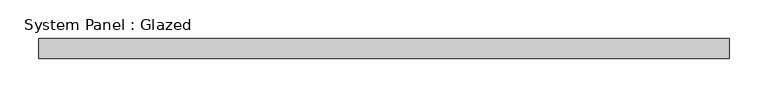
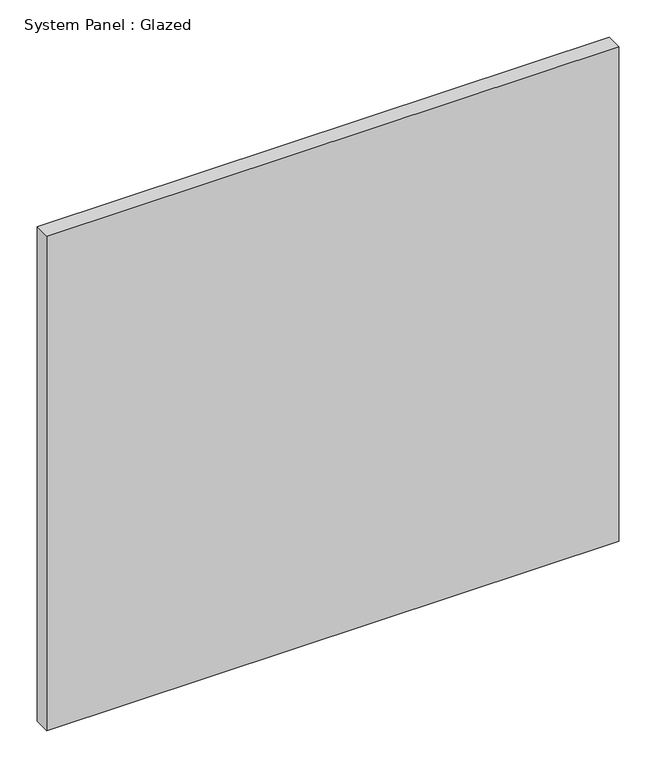
"""IFC4 building model written with IfcOpenShell, lengths in millimetres: plate geometry, System Panel : Glazed."""

import ifcopenshell
import ifcopenshell.guid

model = None  # the IFC model being written
_history = None  # IfcOwnerHistory: only IFC2X3 demands one
_inside = {}  # id of a spatial element -> (the spatial element, [elements in it])
_under = {}  # id of a project, library or spatial element -> (it, [spatial elements below it])
_declared = {}  # id of a project -> (the project, [libraries it declares])
_typed = {}  # id of a type object -> (the type object, [elements of that type])
_made_of = {}  # id of a material, layer set ... -> (it, [elements and type objects made of it])


def new_model(schema):
    """Start an empty IFC model of exactly this schema.

    Asked for "IFC4X3", IfcOpenShell would pick the latest addendum, in which some entities
    have other attributes; the version numbers below select the first issue.
    IFC2X3 requires an IfcOwnerHistory on every rooted entity: one is made here for all.
    """
    global model, _history
    if schema == "IFC4X3":
        model = ifcopenshell.file(schema_version=(4, 3, 0, 0))
    else:
        model = ifcopenshell.file(schema=schema)
    _inside.clear()
    _under.clear()
    _declared.clear()
    _typed.clear()
    _made_of.clear()
    _history = None
    if model.schema == "IFC2X3":
        org = make("IfcOrganization", Name="unknown")
        user = make(
            "IfcPersonAndOrganization",
            ThePerson=make("IfcPerson", FamilyName="unknown"),
            TheOrganization=org,
        )
        app = make(
            "IfcApplication",
            ApplicationDeveloper=org,
            Version="unknown",
            ApplicationFullName="unknown",
            ApplicationIdentifier="unknown",
        )
        _history = make(
            "IfcOwnerHistory",
            OwningUser=user,
            OwningApplication=app,
            ChangeAction="ADDED",
            CreationDate=0,
        )
    return model


def make(cls, **values):
    """One entity of the class cls with the attributes given. An attribute that is None is left unset."""
    return model.create_entity(
        cls, **{name: value for name, value in values.items() if value is not None}
    )


def rooted(cls, **values):
    """An entity with a GlobalId (a new one), such as an element, a storey or a relation."""
    return make(cls, GlobalId=ifcopenshell.guid.new(), OwnerHistory=_history, **values)


def si_unit(unit_type, name, prefix=None):
    """IfcSIUnit, for example si_unit("LENGTHUNIT", "METRE", prefix="MILLI")."""
    return make("IfcSIUnit", UnitType=unit_type, Prefix=prefix, Name=name)


def assignment(units):
    """IfcUnitAssignment: the units of a project."""
    return None if units is None else make("IfcUnitAssignment", Units=units)


def point(xyz):
    """IfcCartesianPoint."""
    return None if xyz is None else make("IfcCartesianPoint", Coordinates=xyz)


def direction(xyz):
    """IfcDirection."""
    return None if xyz is None else make("IfcDirection", DirectionRatios=xyz)


def frame(location, z_axis=None, x_axis=None):
    """IfcAxis2Placement3D, a coordinate frame: its origin and axes. An axis left out is left unset."""
    return make(
        "IfcAxis2Placement3D",
        Location=point(location),
        Axis=direction(z_axis),
        RefDirection=direction(x_axis),
    )


def origin():
    """The frame at (0, 0, 0) with its axes left unset."""
    return frame((0.0, 0.0, 0.0))


def origin_with_axes():
    """The frame at (0, 0, 0) with the z axis (0, 0, 1) and the x axis (1, 0, 0) written out."""
    return frame((0.0, 0.0, 0.0), z_axis=(0.0, 0.0, 1.0), x_axis=(1.0, 0.0, 0.0))


def place(relative_to, where):
    """IfcLocalPlacement: puts the frame where relative to a parent placement (None: the world)."""
    return make(
        "IfcLocalPlacement", PlacementRelTo=relative_to, RelativePlacement=where
    )


def context(
    kind, dimensions, precision=None, world=None, true_north=None, identifier=None
):
    """IfcGeometricRepresentationContext, for example the 3D "Model" context."""
    return make(
        "IfcGeometricRepresentationContext",
        ContextIdentifier=identifier,
        ContextType=kind,
        CoordinateSpaceDimension=dimensions,
        Precision=precision,
        WorldCoordinateSystem=world,
        TrueNorth=true_north,
    )


def project(units=None, contexts=None):
    """IfcProject with its units and contexts."""
    return rooted(
        "IfcProject",
        Name="project",
        RepresentationContexts=contexts,
        UnitsInContext=assignment(units),
    )


def spatial(cls, under=None, at=None, **own):
    """A site, building, storey or space (cls), placed at a placement, below another one or the project."""
    s = rooted(cls, ObjectPlacement=at, **own)
    if under is not None:
        _under.setdefault(under.id(), (under, []))[1].append(s)
    return s


def polyline(points):
    """IfcPolyline through the points."""
    return make("IfcPolyline", Points=[point(p) for p in points])


def outline(outer, holes=None, kind="AREA"):
    """IfcArbitraryClosedProfileDef: a profile drawn as a closed curve; with holes, ...WithVoids."""
    if holes is None:
        return make("IfcArbitraryClosedProfileDef", ProfileType=kind, OuterCurve=outer)
    return make(
        "IfcArbitraryProfileDefWithVoids",
        ProfileType=kind,
        OuterCurve=outer,
        InnerCurves=holes,
    )


def extrude(swept, where, along, depth):
    """IfcExtrudedAreaSolid: the profile swept, set in the frame where, extruded along a direction by depth."""
    return make(
        "IfcExtrudedAreaSolid",
        SweptArea=swept,
        Position=where,
        ExtrudedDirection=direction(along),
        Depth=depth,
    )


def shape(context_of_items, identifier, shape_type, items):
    """IfcShapeRepresentation: the items that make up one representation, for example the "Body"."""
    return make(
        "IfcShapeRepresentation",
        ContextOfItems=context_of_items,
        RepresentationIdentifier=identifier,
        RepresentationType=shape_type,
        Items=items,
    )


def source(mapping_origin, context_of_items, identifier, shape_type, items):
    """IfcRepresentationMap: a shape defined once, which mapped items show again and again."""
    return make(
        "IfcRepresentationMap",
        MappingOrigin=mapping_origin,
        MappedRepresentation=shape(context_of_items, identifier, shape_type, items),
    )


def transform(
    local_origin,
    x_axis=None,
    y_axis=None,
    z_axis=None,
    scale=None,
    scale2=None,
    scale3=None,
    uniform=True,
):
    """IfcCartesianTransformationOperator3D, or its non-uniform kind. x_axis, y_axis, z_axis: its Axis1, 2, 3."""
    if uniform:
        return make(
            "IfcCartesianTransformationOperator3D",
            Axis1=direction(x_axis),
            Axis2=direction(y_axis),
            LocalOrigin=point(local_origin),
            Scale=scale,
            Axis3=direction(z_axis),
        )
    return make(
        "IfcCartesianTransformationOperator3DnonUniform",
        Axis1=direction(x_axis),
        Axis2=direction(y_axis),
        LocalOrigin=point(local_origin),
        Scale=scale,
        Axis3=direction(z_axis),
        Scale2=scale2,
        Scale3=scale3,
    )


def mapped(mapping_source, mapping_target):
    """IfcMappedItem: shows the shape of a source again, moved by a transform."""
    return make(
        "IfcMappedItem", MappingSource=mapping_source, MappingTarget=mapping_target
    )


def made_of(thing, what):
    """Note that an element or type object is made of a material, layer set ...; save() writes the relation."""
    if what is not None:
        _made_of.setdefault(what.id(), (what, []))[1].append(thing)
    return thing


def element(
    cls,
    number,
    at=None,
    inside=None,
    cuts=None,
    type_object=None,
    material=None,
    context=None,
    identifier="Body",
    shape_type=None,
    held_by="IfcProductDefinitionShape",
    body=None,
    shapes=None,
    **own,
):
    """One element of the class cls, such as IfcWall. Its Tag is "e" and its number.

    at: its placement. inside: the storey or other place that contains it. cuts: it is an
    opening in that element (IfcRelVoidsElement). A single representation is given by context,
    identifier, shape_type and body (its items); several are given by shapes. held_by: the class
    of the entity that holds the representations. save() writes the other relations.
    """
    e = rooted(cls, Tag="e%d" % number, ObjectPlacement=at, **own)
    if body is not None:
        shapes = [shape(context, identifier, shape_type, body)]
    if shapes is not None:
        e.Representation = make(held_by, Representations=shapes)
    if inside is not None:
        _inside.setdefault(inside.id(), (inside, []))[1].append(e)
    if cuts is not None:
        rooted(
            "IfcRelVoidsElement", RelatingBuildingElement=cuts, RelatedOpeningElement=e
        )
    if type_object is not None:
        _typed.setdefault(type_object.id(), (type_object, []))[1].append(e)
    return made_of(e, material)


def aggregate(whole, parts):
    """IfcRelAggregates: a whole, such as a stair, and the parts it consists of."""
    return rooted("IfcRelAggregates", RelatingObject=whole, RelatedObjects=parts)


def save(model, path):
    """Write the relations noted so far, then the file.

    IfcRelAggregates (storeys below a building ...), IfcRelContainedInSpatialStructure (elements
    in a storey), IfcRelDefinesByType, IfcRelAssociatesMaterial and IfcRelDeclares: one each for
    every whole, place, type object, material and project.
    """
    for whole, parts in _under.values():
        aggregate(whole, parts)
    for where, things in _inside.values():
        rooted(
            "IfcRelContainedInSpatialStructure",
            RelatedElements=things,
            RelatingStructure=where,
        )
    for kind, things in _typed.values():
        rooted("IfcRelDefinesByType", RelatedObjects=things, RelatingType=kind)
    for what, things in _made_of.values():
        rooted("IfcRelAssociatesMaterial", RelatedObjects=things, RelatingMaterial=what)
    for by, libraries in _declared.values():
        rooted("IfcRelDeclares", RelatingContext=by, RelatedDefinitions=libraries)
    model.write(path)


def system_panel_glazed_bd04319c(model_context):
    return source(origin(), model_context, "Body", "SweptSolid", [
        extrude(outline(polyline([(444.4999998, -44.45), (-444.4999998, -44.45), (-444.4999998, -19.05), (444.4999998, -19.05), (444.4999998, -44.45)])), origin_with_axes(), (0.0, 0.0, 1.0), 812.8),
    ])


if __name__ == "__main__":
    model = new_model("IFC4")
    model_context = context("Model", 3, world=origin())
    ifc_project = project(units=[si_unit("LENGTHUNIT", "METRE", prefix="MILLI")], contexts=[model_context])
    site = spatial("IfcSite", under=ifc_project)
    building = spatial("IfcBuilding", under=site)
    placement = place(None, origin())
    system_panel_glazed_shape = system_panel_glazed_bd04319c(model_context)
    element("IfcPlate", 1, ObjectType="System Panel : Glazed", at=placement, inside=building, context=model_context, shape_type="MappedRepresentation", body=[
        mapped(system_panel_glazed_shape, transform((0.0, 0.0, 0.0), x_axis=(1.0, 0.0, 0.0), y_axis=(0.0, 1.0, 0.0), z_axis=(0.0, 0.0, 1.0))),
    ])
    save(model, "model.ifc")

# Revit data of these elements
# Element 1 (IfcPlate, "System Panel : Glazed")
#   Materials on its faces: "Glass"
# Materials
#   "Glass": class "Glass", colour RGB 0 128 192, transparency 0.75
